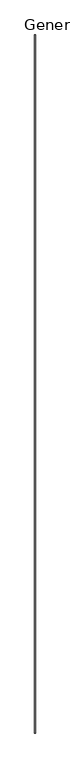
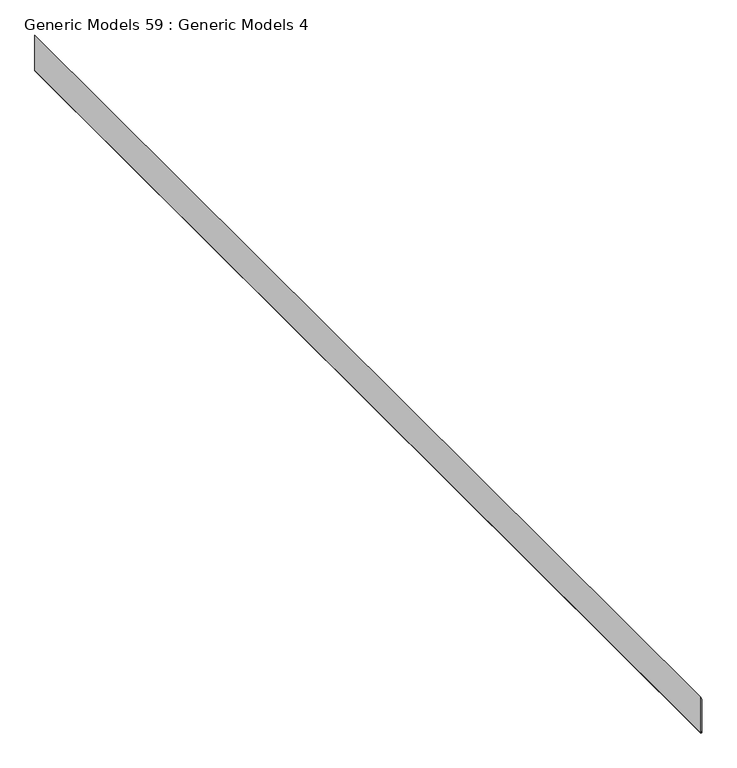
"""IFC4 building model written with IfcOpenShell, lengths in millimetres: proxy geometry, Generic Models 59 : Generic Models 4."""

from ifc_helpers import new_model, si_unit, frame, origin, place, context, project, spatial, polyline, outline, extrude, source, transform, mapped, element, save


def generic_models_59_generic_models_4_d3059ba5(model_context):
    return source(origin(), model_context, "Body", "SweptSolid", [
        extrude(outline(polyline([(126343.791, -9443.8936296), (126918.8908545, -9443.8936296), (126953.515065, -9461.6736296), (126347.2708, -9461.6736296), (126347.2708, -9460.8147887), (126366.3153787, -9460.8147887), (126366.3153787, -9459.5447887), (126346.0008, -9459.5447887), (126346.0008, -9460.4036296), (126343.791, -9460.4036296), (126343.791, -9443.8936296)])), frame((0.0, -6864.9230338, 0.0), z_axis=(0.0, 1.0, 0.0), x_axis=(0.0, 0.0, 1.0)), (0.0, 0.0, 1.0), 18643.6),
    ])


if __name__ == "__main__":
    model = new_model("IFC4")
    model_context = context("Model", 3, world=origin())
    ifc_project = project(units=[si_unit("LENGTHUNIT", "METRE", prefix="MILLI")], contexts=[model_context])
    site = spatial("IfcSite", under=ifc_project)
    building = spatial("IfcBuilding", under=site)
    placement = place(None, origin())
    generic_models_59_generic_models_4_shape = generic_models_59_generic_models_4_d3059ba5(model_context)
    element("IfcBuildingElementProxy", 1, Name="Generic Models 59 : Generic Models 4", ObjectType="Generic Models 59 : Generic Models 4", at=placement, inside=building, context=model_context, shape_type="MappedRepresentation", body=[
        mapped(generic_models_59_generic_models_4_shape, transform((0.0, 0.0, 0.0), x_axis=(1.0, 0.0, 0.0), y_axis=(0.0, 1.0, 0.0), z_axis=(0.0, 0.0, 1.0))),
    ])
    save(model, "model.ifc")

# Revit data of these elements
# Element 1 (IfcBuildingElementProxy, "Generic Models 59 : Generic Models 4")
#   Materials on its faces: "_7/8\" SMOOTH TROWEL EXTERIOR STUCCO (COLOR PER OWNER)"
# Materials
#   "_7/8\" SMOOTH TROWEL EXTERIOR STUCCO (COLOR PER OWNER)": class "Generic", colour RGB 233 233 233, transparency 0, Cost = 0
